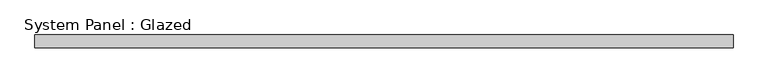
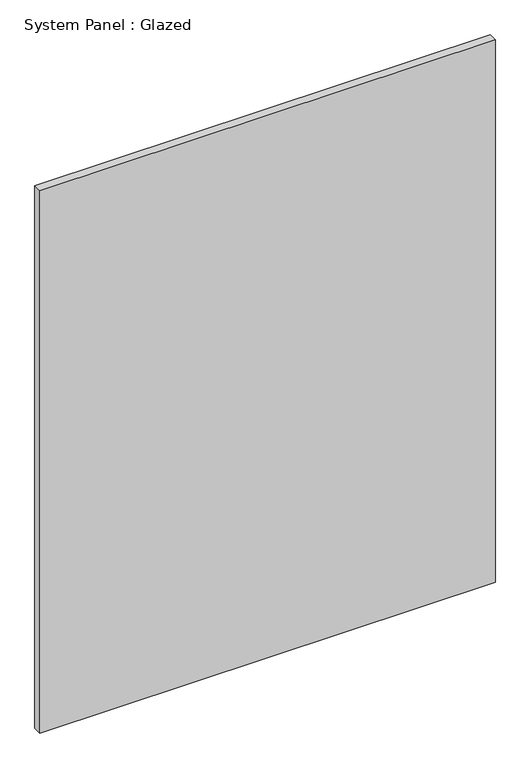
"""IFC4 building model written with IfcOpenShell, lengths in millimetres: plate geometry, System Panel : Glazed."""

from ifc_helpers import new_model, si_unit, origin, origin_with_axes, place, context, project, spatial, polyline, outline, extrude, source, transform, mapped, element, save


def system_panel_glazed_b5691209(model_context):
    return source(origin(), model_context, "Body", "SweptSolid", [
        extrude(outline(polyline([(669.9999998, 24.5), (-669.9999998, 24.5), (-669.9999998, 49.5), (669.9999998, 49.5), (669.9999998, 24.5)])), origin_with_axes(), (0.0, 0.0, 1.0), 1686.2355347),
    ])


if __name__ == "__main__":
    model = new_model("IFC4")
    model_context = context("Model", 3, world=origin())
    ifc_project = project(units=[si_unit("LENGTHUNIT", "METRE", prefix="MILLI")], contexts=[model_context])
    site = spatial("IfcSite", under=ifc_project)
    building = spatial("IfcBuilding", under=site)
    placement = place(None, origin())
    system_panel_glazed_shape = system_panel_glazed_b5691209(model_context)
    element("IfcPlate", 1, ObjectType="System Panel : Glazed", at=placement, inside=building, context=model_context, shape_type="MappedRepresentation", body=[
        mapped(system_panel_glazed_shape, transform((0.0, 0.0, 0.0), x_axis=(1.0, 0.0, 0.0), y_axis=(0.0, 1.0, 0.0), z_axis=(0.0, 0.0, 1.0))),
    ])
    save(model, "model.ifc")

# Revit data of these elements
# Element 1 (IfcPlate, "System Panel : Glazed")
#   Materials on its faces: "Glass"
# Materials
#   "Glass": class "Glass", colour RGB 218 227 224, transparency 0.85, Description = "Soda Lime Glass", Cost = 0
